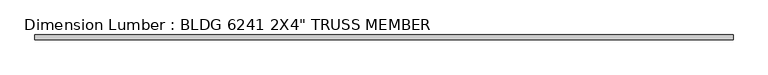
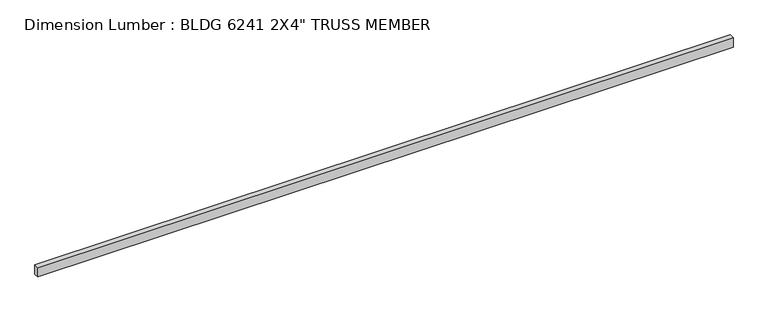
"""IFC4 building model written with IfcOpenShell, lengths in millimetres: beam geometry."""

import ifcopenshell
import ifcopenshell.guid

model = None  # the IFC model being written
_history = None  # IfcOwnerHistory: only IFC2X3 demands one
_inside = {}  # id of a spatial element -> (the spatial element, [elements in it])
_under = {}  # id of a project, library or spatial element -> (it, [spatial elements below it])
_declared = {}  # id of a project -> (the project, [libraries it declares])
_typed = {}  # id of a type object -> (the type object, [elements of that type])
_made_of = {}  # id of a material, layer set ... -> (it, [elements and type objects made of it])


def new_model(schema):
    """Start an empty IFC model of exactly this schema.

    Asked for "IFC4X3", IfcOpenShell would pick the latest addendum, in which some entities
    have other attributes; the version numbers below select the first issue.
    IFC2X3 requires an IfcOwnerHistory on every rooted entity: one is made here for all.
    """
    global model, _history
    if schema == "IFC4X3":
        model = ifcopenshell.file(schema_version=(4, 3, 0, 0))
    else:
        model = ifcopenshell.file(schema=schema)
    _inside.clear()
    _under.clear()
    _declared.clear()
    _typed.clear()
    _made_of.clear()
    _history = None
    if model.schema == "IFC2X3":
        org = make("IfcOrganization", Name="unknown")
        user = make(
            "IfcPersonAndOrganization",
            ThePerson=make("IfcPerson", FamilyName="unknown"),
            TheOrganization=org,
        )
        app = make(
            "IfcApplication",
            ApplicationDeveloper=org,
            Version="unknown",
            ApplicationFullName="unknown",
            ApplicationIdentifier="unknown",
        )
        _history = make(
            "IfcOwnerHistory",
            OwningUser=user,
            OwningApplication=app,
            ChangeAction="ADDED",
            CreationDate=0,
        )
    return model


def make(cls, **values):
    """One entity of the class cls with the attributes given. An attribute that is None is left unset."""
    return model.create_entity(
        cls, **{name: value for name, value in values.items() if value is not None}
    )


def rooted(cls, **values):
    """An entity with a GlobalId (a new one), such as an element, a storey or a relation."""
    return make(cls, GlobalId=ifcopenshell.guid.new(), OwnerHistory=_history, **values)


def si_unit(unit_type, name, prefix=None):
    """IfcSIUnit, for example si_unit("LENGTHUNIT", "METRE", prefix="MILLI")."""
    return make("IfcSIUnit", UnitType=unit_type, Prefix=prefix, Name=name)


def assignment(units):
    """IfcUnitAssignment: the units of a project."""
    return None if units is None else make("IfcUnitAssignment", Units=units)


def point(xyz):
    """IfcCartesianPoint."""
    return None if xyz is None else make("IfcCartesianPoint", Coordinates=xyz)


def direction(xyz):
    """IfcDirection."""
    return None if xyz is None else make("IfcDirection", DirectionRatios=xyz)


def frame(location, z_axis=None, x_axis=None):
    """IfcAxis2Placement3D, a coordinate frame: its origin and axes. An axis left out is left unset."""
    return make(
        "IfcAxis2Placement3D",
        Location=point(location),
        Axis=direction(z_axis),
        RefDirection=direction(x_axis),
    )


def origin():
    """The frame at (0, 0, 0) with its axes left unset."""
    return frame((0.0, 0.0, 0.0))


def place(relative_to, where):
    """IfcLocalPlacement: puts the frame where relative to a parent placement (None: the world)."""
    return make(
        "IfcLocalPlacement", PlacementRelTo=relative_to, RelativePlacement=where
    )


def context(
    kind, dimensions, precision=None, world=None, true_north=None, identifier=None
):
    """IfcGeometricRepresentationContext, for example the 3D "Model" context."""
    return make(
        "IfcGeometricRepresentationContext",
        ContextIdentifier=identifier,
        ContextType=kind,
        CoordinateSpaceDimension=dimensions,
        Precision=precision,
        WorldCoordinateSystem=world,
        TrueNorth=true_north,
    )


def project(units=None, contexts=None):
    """IfcProject with its units and contexts."""
    return rooted(
        "IfcProject",
        Name="project",
        RepresentationContexts=contexts,
        UnitsInContext=assignment(units),
    )


def spatial(cls, under=None, at=None, **own):
    """A site, building, storey or space (cls), placed at a placement, below another one or the project."""
    s = rooted(cls, ObjectPlacement=at, **own)
    if under is not None:
        _under.setdefault(under.id(), (under, []))[1].append(s)
    return s


def polyline(points):
    """IfcPolyline through the points."""
    return make("IfcPolyline", Points=[point(p) for p in points])


def outline(outer, holes=None, kind="AREA"):
    """IfcArbitraryClosedProfileDef: a profile drawn as a closed curve; with holes, ...WithVoids."""
    if holes is None:
        return make("IfcArbitraryClosedProfileDef", ProfileType=kind, OuterCurve=outer)
    return make(
        "IfcArbitraryProfileDefWithVoids",
        ProfileType=kind,
        OuterCurve=outer,
        InnerCurves=holes,
    )


def extrude(swept, where, along, depth):
    """IfcExtrudedAreaSolid: the profile swept, set in the frame where, extruded along a direction by depth."""
    return make(
        "IfcExtrudedAreaSolid",
        SweptArea=swept,
        Position=where,
        ExtrudedDirection=direction(along),
        Depth=depth,
    )


def shape(context_of_items, identifier, shape_type, items):
    """IfcShapeRepresentation: the items that make up one representation, for example the "Body"."""
    return make(
        "IfcShapeRepresentation",
        ContextOfItems=context_of_items,
        RepresentationIdentifier=identifier,
        RepresentationType=shape_type,
        Items=items,
    )


def source(mapping_origin, context_of_items, identifier, shape_type, items):
    """IfcRepresentationMap: a shape defined once, which mapped items show again and again."""
    return make(
        "IfcRepresentationMap",
        MappingOrigin=mapping_origin,
        MappedRepresentation=shape(context_of_items, identifier, shape_type, items),
    )


def transform(
    local_origin,
    x_axis=None,
    y_axis=None,
    z_axis=None,
    scale=None,
    scale2=None,
    scale3=None,
    uniform=True,
):
    """IfcCartesianTransformationOperator3D, or its non-uniform kind. x_axis, y_axis, z_axis: its Axis1, 2, 3."""
    if uniform:
        return make(
            "IfcCartesianTransformationOperator3D",
            Axis1=direction(x_axis),
            Axis2=direction(y_axis),
            LocalOrigin=point(local_origin),
            Scale=scale,
            Axis3=direction(z_axis),
        )
    return make(
        "IfcCartesianTransformationOperator3DnonUniform",
        Axis1=direction(x_axis),
        Axis2=direction(y_axis),
        LocalOrigin=point(local_origin),
        Scale=scale,
        Axis3=direction(z_axis),
        Scale2=scale2,
        Scale3=scale3,
    )


def mapped(mapping_source, mapping_target):
    """IfcMappedItem: shows the shape of a source again, moved by a transform."""
    return make(
        "IfcMappedItem", MappingSource=mapping_source, MappingTarget=mapping_target
    )


def made_of(thing, what):
    """Note that an element or type object is made of a material, layer set ...; save() writes the relation."""
    if what is not None:
        _made_of.setdefault(what.id(), (what, []))[1].append(thing)
    return thing


def element(
    cls,
    number,
    at=None,
    inside=None,
    cuts=None,
    type_object=None,
    material=None,
    context=None,
    identifier="Body",
    shape_type=None,
    held_by="IfcProductDefinitionShape",
    body=None,
    shapes=None,
    **own,
):
    """One element of the class cls, such as IfcWall. Its Tag is "e" and its number.

    at: its placement. inside: the storey or other place that contains it. cuts: it is an
    opening in that element (IfcRelVoidsElement). A single representation is given by context,
    identifier, shape_type and body (its items); several are given by shapes. held_by: the class
    of the entity that holds the representations. save() writes the other relations.
    """
    e = rooted(cls, Tag="e%d" % number, ObjectPlacement=at, **own)
    if body is not None:
        shapes = [shape(context, identifier, shape_type, body)]
    if shapes is not None:
        e.Representation = make(held_by, Representations=shapes)
    if inside is not None:
        _inside.setdefault(inside.id(), (inside, []))[1].append(e)
    if cuts is not None:
        rooted(
            "IfcRelVoidsElement", RelatingBuildingElement=cuts, RelatedOpeningElement=e
        )
    if type_object is not None:
        _typed.setdefault(type_object.id(), (type_object, []))[1].append(e)
    return made_of(e, material)


def aggregate(whole, parts):
    """IfcRelAggregates: a whole, such as a stair, and the parts it consists of."""
    return rooted("IfcRelAggregates", RelatingObject=whole, RelatedObjects=parts)


def save(model, path):
    """Write the relations noted so far, then the file.

    IfcRelAggregates (storeys below a building ...), IfcRelContainedInSpatialStructure (elements
    in a storey), IfcRelDefinesByType, IfcRelAssociatesMaterial and IfcRelDeclares: one each for
    every whole, place, type object, material and project.
    """
    for whole, parts in _under.values():
        aggregate(whole, parts)
    for where, things in _inside.values():
        rooted(
            "IfcRelContainedInSpatialStructure",
            RelatedElements=things,
            RelatingStructure=where,
        )
    for kind, things in _typed.values():
        rooted("IfcRelDefinesByType", RelatedObjects=things, RelatingType=kind)
    for what, things in _made_of.values():
        rooted("IfcRelAssociatesMaterial", RelatedObjects=things, RelatingMaterial=what)
    for by, libraries in _declared.values():
        rooted("IfcRelDeclares", RelatingContext=by, RelatedDefinitions=libraries)
    model.write(path)


def beam_44bcd8c2(model_context):
    return source(origin(), model_context, "Body", "SweptSolid", [
        extrude(outline(polyline([(3555.9999994, 25.4), (3555.9999994, -25.4), (-3555.9999994, -25.4), (-3555.9999994, 25.4), (3555.9999994, 25.4)])), frame((0.0, 0.0, -50.8), z_axis=(0.0, 0.0, 1.0), x_axis=(1.0, 0.0, 0.0)), (0.0, 0.0, 1.0), 101.6),
    ])


if __name__ == "__main__":
    model = new_model("IFC4")
    model_context = context("Model", 3, world=origin())
    ifc_project = project(units=[si_unit("LENGTHUNIT", "METRE", prefix="MILLI")], contexts=[model_context])
    site = spatial("IfcSite", under=ifc_project)
    building = spatial("IfcBuilding", under=site)
    placement = place(None, origin())
    beam_shape = beam_44bcd8c2(model_context)
    element("IfcBeam", 1, ObjectType="Dimension Lumber : BLDG 6241 2X4\" TRUSS MEMBER", at=placement, inside=building, context=model_context, shape_type="MappedRepresentation", body=[
        mapped(beam_shape, transform((0.0, 0.0, 0.0), x_axis=(1.0, 0.0, 0.0), y_axis=(0.0, 1.0, 0.0), z_axis=(0.0, 0.0, 1.0))),
    ])
    save(model, "model.ifc")

# Revit data of these elements
# Type "Dimension Lumber : BLDG 6241 2X4\" TRUSS MEMBER"
#   Assembly Code = "B10"
#   A = 0.273472 SF
#   Length [instance default] = 5' - 0"
#   b = 0' - 2"
#   d = 0' - 4"
#   Structural Material [instance default] = Softwood, Lumber
# Element 1 (IfcBeam, "Dimension Lumber : BLDG 6241 2X4\" TRUSS MEMBER")
#   Materials on its faces: "Softwood, Lumber"
# Materials
#   "Softwood, Lumber": class "Wood", colour RGB 223 192 134, transparency 0, Description = "Pinus Echinata", Cost = 0
